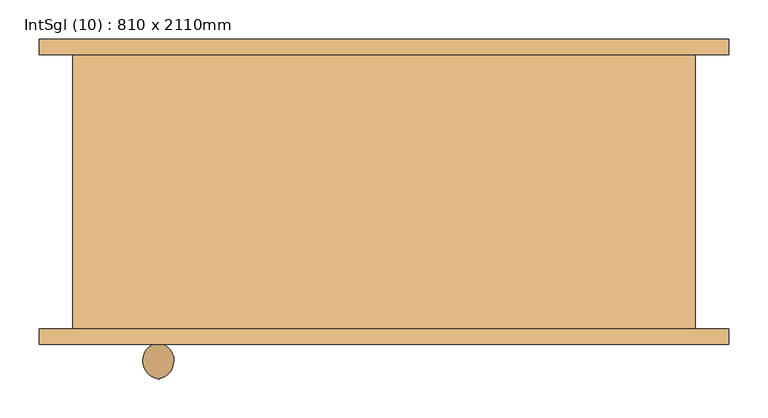
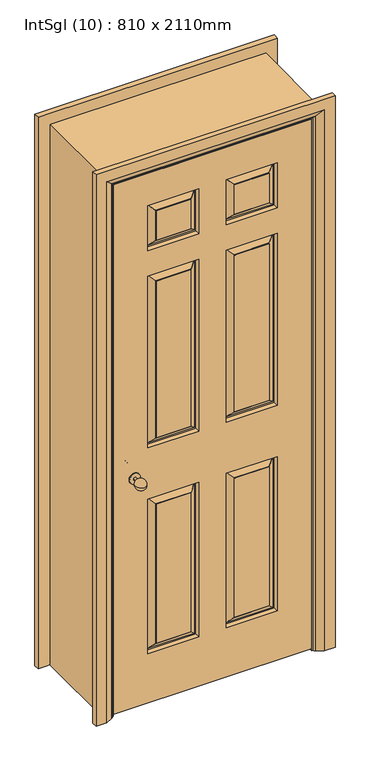
"""IFC4 building model written with IfcOpenShell, lengths in millimetres: door geometry, IntSgl (10) : 810 x 2110mm."""

from ifc_helpers import new_model, si_unit, point, frame, origin, place, context, project, spatial, polyline, circle_curve, ellipse_curve, trimmed, outline, extrude, faceted_brep, source, transform, mapped, element, save
from ifc_brep_helpers import plane_surface, cylinder_surface, revolved_surface, advanced_brep


def intsgl_10_810_x_2110mm_217d45f9(model_context):
    return source(origin(), model_context, "Body", "SolidModel", [
        advanced_brep(
        [(-283.0, -118.0, 900.0), (-293.0, -118.0, 900.0), (-288.0, -73.562589, 900.0), (-283.0, -133.0, 900.0), (-293.0, -133.0, 900.0), (-308.0, -137.0, 900.0), (-268.0, -137.0, 900.0), (-308.0, -133.0, 900.0), (-268.0, -133.0, 900.0)],
        [
            (0, 1, circle_curve(frame((-288.0, -118.0, 900.0), z_axis=(0.0, 1.0, 0.0), x_axis=(-1.0, 0.0, 0.0)), 5.0)),
            (1, 2, circle_curve(frame((-284.8115138, -96.4213505, 900.0), z_axis=(0.0, 0.0, -1.0), x_axis=(0.0, -1.0, 0.0)), 23.0800654)),
            (2, 0, circle_curve(frame((-291.1884862, -96.4213505, 900.0), z_axis=(0.0, 0.0, -1.0), x_axis=(0.0, -1.0, 0.0)), 23.0800654)),
            (1, 0, circle_curve(frame((-288.0, -118.0, 900.0), z_axis=(0.0, 1.0, 0.0), x_axis=(-1.0, 0.0, 0.0)), 5.0)),
            (0, 3),
            (3, 4, circle_curve(frame((-288.0, -133.0, 900.0), z_axis=(0.0, 1.0, 0.0), x_axis=(-1.0, 0.0, 0.0)), 5.0)),
            (4, 1),
            (4, 3, circle_curve(frame((-288.0, -133.0, 900.0), z_axis=(0.0, 1.0, 0.0), x_axis=(-1.0, 0.0, 0.0)), 5.0)),
            (5, 6, circle_curve(frame((-288.0, -137.0, 900.0), z_axis=(0.0, -1.0, 0.0), x_axis=(1.0, 0.0, 0.0)), 20.0)),
            (6, 5, circle_curve(frame((-288.0, -137.0, 900.0), z_axis=(0.0, -1.0, 0.0), x_axis=(1.0, 0.0, 0.0)), 20.0)),
            (7, 8, circle_curve(frame((-288.0, -133.0, 900.0), z_axis=(0.0, 1.0, 0.0), x_axis=(1.0, 0.0, 0.0)), 20.0)),
            (8, 7, circle_curve(frame((-288.0, -133.0, 900.0), z_axis=(0.0, 1.0, 0.0), x_axis=(1.0, 0.0, 0.0)), 20.0)),
            (5, 7),
            (8, 6),
        ],
        [
            revolved_surface(trimmed(ellipse_curve(frame((-284.8115138, -96.4213505, 900.0), z_axis=(0.0, 0.0, 1.0), x_axis=(0.0, -1.0, 0.0)), 23.0800654, 23.0800654), [point((-288.0, -73.562589, 900.0))], [point((-293.0, -118.0, 900.0))], True, "CARTESIAN"), (-288.0, -133.0, 900.0), (0.0, -1.0, 0.0)),
            cylinder_surface(frame((-288.0, -133.0, 900.0), z_axis=(0.0, -1.0, 0.0), x_axis=(-1.0, 0.0, 0.0)), 5.0),
            plane_surface(frame((-268.0, -137.0, 900.0), z_axis=(0.0, -1.0, 0.0), x_axis=(0.0, 0.0, 1.0))),
            plane_surface(frame((-268.0, -133.0, 900.0), z_axis=(0.0, 1.0, 0.0), x_axis=(0.0, 0.0, -1.0))),
            cylinder_surface(frame((-288.0, -133.0, 900.0), z_axis=(0.0, -1.0, 0.0), x_axis=(1.0, 0.0, 0.0)), 20.0),
        ],
        [
            (0, [[1, 2, 3]]),
            (0, [[-2, 4, -3]]),
            (1, [[-1, 5, 6, 7]]),
            (1, [[-4, -7, 8, -5]]),
            (2, [[9, 10]]),
            (3, [[11, 12], [-6, -8]]),
            (4, [[-9, 13, -12, 14]]),
            (4, [[-10, -14, -11, -13]]),
        ],
    ),
        advanced_brep(
        [(-283.0, -194.0, 900.0), (-288.0, -238.437411, 900.0), (-293.0, -194.0, 900.0), (-293.0, -179.0, 900.0), (-283.0, -179.0, 900.0), (-308.0, -175.0, 900.0), (-268.0, -175.0, 900.0), (-308.0, -179.0, 900.0), (-268.0, -179.0, 900.0)],
        [
            (0, 1, circle_curve(frame((-291.1884862, -215.5786495, 900.0), z_axis=(0.0, 0.0, -1.0), x_axis=(0.0, 1.0, 0.0)), 23.0800654)),
            (1, 2, circle_curve(frame((-284.8115138, -215.5786495, 900.0), z_axis=(0.0, 0.0, -1.0), x_axis=(0.0, 1.0, 0.0)), 23.0800654)),
            (2, 0, circle_curve(frame((-288.0, -194.0, 900.0), z_axis=(0.0, -1.0, 0.0), x_axis=(-1.0, 0.0, 0.0)), 5.0)),
            (0, 2, circle_curve(frame((-288.0, -194.0, 900.0), z_axis=(0.0, -1.0, 0.0), x_axis=(-1.0, 0.0, 0.0)), 5.0)),
            (2, 3),
            (3, 4, circle_curve(frame((-288.0, -179.0, 900.0), z_axis=(0.0, -1.0, 0.0), x_axis=(-1.0, 0.0, 0.0)), 5.0)),
            (4, 0),
            (4, 3, circle_curve(frame((-288.0, -179.0, 900.0), z_axis=(0.0, -1.0, 0.0), x_axis=(-1.0, 0.0, 0.0)), 5.0)),
            (5, 6, circle_curve(frame((-288.0, -175.0, 900.0), z_axis=(0.0, 1.0, 0.0), x_axis=(1.0, 0.0, 0.0)), 20.0)),
            (6, 5, circle_curve(frame((-288.0, -175.0, 900.0), z_axis=(0.0, 1.0, 0.0), x_axis=(1.0, 0.0, 0.0)), 20.0)),
            (7, 8, circle_curve(frame((-288.0, -179.0, 900.0), z_axis=(0.0, -1.0, 0.0), x_axis=(1.0, 0.0, 0.0)), 20.0)),
            (8, 7, circle_curve(frame((-288.0, -179.0, 900.0), z_axis=(0.0, -1.0, 0.0), x_axis=(1.0, 0.0, 0.0)), 20.0)),
            (6, 8),
            (7, 5),
        ],
        [
            revolved_surface(trimmed(ellipse_curve(frame((-284.8115138, -215.5786495, 900.0), z_axis=(0.0, 0.0, -1.0), x_axis=(0.0, 1.0, 0.0)), 23.0800654, 23.0800654), [point((-288.0, -238.437411, 900.0))], [point((-293.0, -194.0, 900.0))], True, "CARTESIAN"), (-288.0, -179.0, 900.0), (0.0, 1.0, 0.0)),
            cylinder_surface(frame((-288.0, -179.0, 900.0), z_axis=(0.0, 1.0, 0.0), x_axis=(-1.0, 0.0, 0.0)), 5.0),
            plane_surface(frame((-268.0, -175.0, 900.0), z_axis=(0.0, 1.0, 0.0), x_axis=(0.0, 0.0, 1.0))),
            plane_surface(frame((-268.0, -179.0, 900.0), z_axis=(0.0, -1.0, 0.0), x_axis=(0.0, 0.0, -1.0))),
            cylinder_surface(frame((-288.0, -179.0, 900.0), z_axis=(0.0, 1.0, 0.0), x_axis=(1.0, 0.0, 0.0)), 20.0),
        ],
        [
            (0, [[1, 2, 3]]),
            (0, [[-1, 4, -2]]),
            (1, [[5, 6, 7, -3]]),
            (1, [[-7, 8, -5, -4]]),
            (2, [[9, 10]]),
            (3, [[11, 12], [-8, -6]]),
            (4, [[13, -11, 14, -10]]),
            (4, [[-14, -12, -13, -9]]),
        ],
    ),
        faceted_brep([(-363.0, -137.0, 2068.0), (363.0, -137.0, 2068.0), (363.0, -137.0, 8.0), (-363.0, -137.0, 8.0), (-50.0, -137.0, 800.0), (-238.0, -137.0, 800.0), (-238.0, -137.0, 200.0), (-50.0, -137.0, 200.0), (238.0, -137.0, 800.0), (50.0, -137.0, 800.0), (50.0, -137.0, 200.0), (238.0, -137.0, 200.0), (-50.0, -137.0, 1668.0), (-238.0, -137.0, 1668.0), (-238.0, -137.0, 1000.0), (-50.0, -137.0, 1000.0), (238.0, -137.0, 1668.0), (50.0, -137.0, 1668.0), (50.0, -137.0, 1000.0), (238.0, -137.0, 1000.0), (-50.0, -137.0, 1943.0), (-238.0, -137.0, 1943.0), (-238.0, -137.0, 1768.0), (-50.0, -137.0, 1768.0), (238.0, -137.0, 1943.0), (50.0, -137.0, 1943.0), (50.0, -137.0, 1768.0), (238.0, -137.0, 1768.0), (-80.0, -137.0, 230.0), (-208.0, -137.0, 230.0), (-208.0, -137.0, 770.0), (-80.0, -137.0, 770.0), (208.0, -137.0, 230.0), (80.0, -137.0, 230.0), (80.0, -137.0, 770.0), (208.0, -137.0, 770.0), (-80.0, -137.0, 1030.0), (-208.0, -137.0, 1030.0), (-208.0, -137.0, 1638.0), (-80.0, -137.0, 1638.0), (208.0, -137.0, 1030.0), (80.0, -137.0, 1030.0), (80.0, -137.0, 1638.0), (208.0, -137.0, 1638.0), (-80.0, -137.0, 1798.0), (-208.0, -137.0, 1798.0), (-208.0, -137.0, 1913.0), (-80.0, -137.0, 1913.0), (208.0, -137.0, 1798.0), (80.0, -137.0, 1798.0), (80.0, -137.0, 1913.0), (208.0, -137.0, 1913.0), (-363.0, -175.0, 2068.0), (-363.0, -175.0, 8.0), (363.0, -175.0, 8.0), (363.0, -175.0, 2068.0), (50.0, -175.0, 800.0), (238.0, -175.0, 800.0), (238.0, -175.0, 200.0), (50.0, -175.0, 200.0), (-238.0, -175.0, 800.0), (-50.0, -175.0, 800.0), (-50.0, -175.0, 200.0), (-238.0, -175.0, 200.0), (50.0, -175.0, 1668.0), (238.0, -175.0, 1668.0), (238.0, -175.0, 1000.0), (50.0, -175.0, 1000.0), (-238.0, -175.0, 1668.0), (-50.0, -175.0, 1668.0), (-50.0, -175.0, 1000.0), (-238.0, -175.0, 1000.0), (50.0, -175.0, 1943.0), (238.0, -175.0, 1943.0), (238.0, -175.0, 1768.0), (50.0, -175.0, 1768.0), (-238.0, -175.0, 1943.0), (-50.0, -175.0, 1943.0), (-50.0, -175.0, 1768.0), (-238.0, -175.0, 1768.0), (80.0, -175.0, 230.0), (208.0, -175.0, 230.0), (208.0, -175.0, 770.0), (80.0, -175.0, 770.0), (-208.0, -175.0, 230.0), (-80.0, -175.0, 230.0), (-80.0, -175.0, 770.0), (-208.0, -175.0, 770.0), (80.0, -175.0, 1030.0), (208.0, -175.0, 1030.0), (208.0, -175.0, 1638.0), (80.0, -175.0, 1638.0), (-208.0, -175.0, 1030.0), (-80.0, -175.0, 1030.0), (-80.0, -175.0, 1638.0), (-208.0, -175.0, 1638.0), (80.0, -175.0, 1798.0), (208.0, -175.0, 1798.0), (208.0, -175.0, 1913.0), (80.0, -175.0, 1913.0), (-208.0, -175.0, 1798.0), (-80.0, -175.0, 1798.0), (-80.0, -175.0, 1913.0), (-208.0, -175.0, 1913.0), (80.0, -174.0, 230.0), (80.0, -174.0, 770.0), (58.0, -160.0, 208.0), (78.0, -174.0, 228.0), (78.0, -174.0, 772.0), (58.0, -160.0, 792.0), (53.0, -160.0, 203.0), (53.0, -160.0, 797.0), (208.0, -174.0, 770.0), (210.0, -174.0, 772.0), (230.0, -160.0, 792.0), (235.0, -160.0, 797.0), (208.0, -174.0, 230.0), (210.0, -174.0, 228.0), (230.0, -160.0, 208.0), (235.0, -160.0, 203.0), (-208.0, -174.0, 230.0), (-208.0, -174.0, 770.0), (-230.0, -160.0, 208.0), (-210.0, -174.0, 228.0), (-210.0, -174.0, 772.0), (-230.0, -160.0, 792.0), (-235.0, -160.0, 203.0), (-235.0, -160.0, 797.0), (-80.0, -174.0, 770.0), (-78.0, -174.0, 772.0), (-58.0, -160.0, 792.0), (-53.0, -160.0, 797.0), (-80.0, -174.0, 230.0), (-78.0, -174.0, 228.0), (-58.0, -160.0, 208.0), (-53.0, -160.0, 203.0), (80.0, -174.0, 1030.0), (80.0, -174.0, 1638.0), (58.0, -160.0, 1008.0), (78.0, -174.0, 1028.0), (78.0, -174.0, 1640.0), (58.0, -160.0, 1660.0), (53.0, -160.0, 1003.0), (53.0, -160.0, 1665.0), (208.0, -174.0, 1638.0), (210.0, -174.0, 1640.0), (230.0, -160.0, 1660.0), (235.0, -160.0, 1665.0), (208.0, -174.0, 1030.0), (210.0, -174.0, 1028.0), (230.0, -160.0, 1008.0), (235.0, -160.0, 1003.0), (-208.0, -174.0, 1030.0), (-208.0, -174.0, 1638.0), (-230.0, -160.0, 1008.0), (-210.0, -174.0, 1028.0), (-210.0, -174.0, 1640.0), (-230.0, -160.0, 1660.0), (-235.0, -160.0, 1003.0), (-235.0, -160.0, 1665.0), (-80.0, -174.0, 1638.0), (-78.0, -174.0, 1640.0), (-58.0, -160.0, 1660.0), (-53.0, -160.0, 1665.0), (-80.0, -174.0, 1030.0), (-78.0, -174.0, 1028.0), (-58.0, -160.0, 1008.0), (-53.0, -160.0, 1003.0), (80.0, -174.0, 1798.0), (80.0, -174.0, 1913.0), (58.0, -160.0, 1776.0), (78.0, -174.0, 1796.0), (78.0, -174.0, 1915.0), (58.0, -160.0, 1935.0), (53.0, -160.0, 1771.0), (53.0, -160.0, 1940.0), (208.0, -174.0, 1913.0), (210.0, -174.0, 1915.0), (230.0, -160.0, 1935.0), (235.0, -160.0, 1940.0), (208.0, -174.0, 1798.0), (210.0, -174.0, 1796.0), (230.0, -160.0, 1776.0), (235.0, -160.0, 1771.0), (-208.0, -174.0, 1798.0), (-208.0, -174.0, 1913.0), (-230.0, -160.0, 1776.0), (-210.0, -174.0, 1796.0), (-210.0, -174.0, 1915.0), (-230.0, -160.0, 1935.0), (-235.0, -160.0, 1771.0), (-235.0, -160.0, 1940.0), (-80.0, -174.0, 1913.0), (-78.0, -174.0, 1915.0), (-58.0, -160.0, 1935.0), (-53.0, -160.0, 1940.0), (-80.0, -174.0, 1798.0), (-78.0, -174.0, 1796.0), (-58.0, -160.0, 1776.0), (-53.0, -160.0, 1771.0), (-80.0, -138.0, 230.0), (-80.0, -138.0, 770.0), (-58.0, -152.0, 208.0), (-78.0, -138.0, 228.0), (-78.0, -138.0, 772.0), (-58.0, -152.0, 792.0), (-53.0, -152.0, 203.0), (-53.0, -152.0, 797.0), (-208.0, -138.0, 770.0), (-210.0, -138.0, 772.0), (-230.0, -152.0, 792.0), (-235.0, -152.0, 797.0), (-208.0, -138.0, 230.0), (-210.0, -138.0, 228.0), (-230.0, -152.0, 208.0), (-235.0, -152.0, 203.0), (208.0, -138.0, 230.0), (208.0, -138.0, 770.0), (230.0, -152.0, 208.0), (210.0, -138.0, 228.0), (210.0, -138.0, 772.0), (230.0, -152.0, 792.0), (235.0, -152.0, 203.0), (235.0, -152.0, 797.0), (80.0, -138.0, 770.0), (78.0, -138.0, 772.0), (58.0, -152.0, 792.0), (53.0, -152.0, 797.0), (80.0, -138.0, 230.0), (78.0, -138.0, 228.0), (58.0, -152.0, 208.0), (53.0, -152.0, 203.0), (-80.0, -138.0, 1030.0), (-80.0, -138.0, 1638.0), (-58.0, -152.0, 1008.0), (-78.0, -138.0, 1028.0), (-78.0, -138.0, 1640.0), (-58.0, -152.0, 1660.0), (-53.0, -152.0, 1003.0), (-53.0, -152.0, 1665.0), (-208.0, -138.0, 1638.0), (-210.0, -138.0, 1640.0), (-230.0, -152.0, 1660.0), (-235.0, -152.0, 1665.0), (-208.0, -138.0, 1030.0), (-210.0, -138.0, 1028.0), (-230.0, -152.0, 1008.0), (-235.0, -152.0, 1003.0), (208.0, -138.0, 1030.0), (208.0, -138.0, 1638.0), (230.0, -152.0, 1008.0), (210.0, -138.0, 1028.0), (210.0, -138.0, 1640.0), (230.0, -152.0, 1660.0), (235.0, -152.0, 1003.0), (235.0, -152.0, 1665.0), (80.0, -138.0, 1638.0), (78.0, -138.0, 1640.0), (58.0, -152.0, 1660.0), (53.0, -152.0, 1665.0), (80.0, -138.0, 1030.0), (78.0, -138.0, 1028.0), (58.0, -152.0, 1008.0), (53.0, -152.0, 1003.0), (-80.0, -138.0, 1798.0), (-80.0, -138.0, 1913.0), (-58.0, -152.0, 1776.0), (-78.0, -138.0, 1796.0), (-78.0, -138.0, 1915.0), (-58.0, -152.0, 1935.0), (-53.0, -152.0, 1771.0), (-53.0, -152.0, 1940.0), (-208.0, -138.0, 1913.0), (-210.0, -138.0, 1915.0), (-230.0, -152.0, 1935.0), (-235.0, -152.0, 1940.0), (-208.0, -138.0, 1798.0), (-210.0, -138.0, 1796.0), (-230.0, -152.0, 1776.0), (-235.0, -152.0, 1771.0), (208.0, -138.0, 1798.0), (208.0, -138.0, 1913.0), (230.0, -152.0, 1776.0), (210.0, -138.0, 1796.0), (210.0, -138.0, 1915.0), (230.0, -152.0, 1935.0), (235.0, -152.0, 1771.0), (235.0, -152.0, 1940.0), (80.0, -138.0, 1913.0), (78.0, -138.0, 1915.0), (58.0, -152.0, 1935.0), (53.0, -152.0, 1940.0), (80.0, -138.0, 1798.0), (78.0, -138.0, 1796.0), (58.0, -152.0, 1776.0), (53.0, -152.0, 1771.0)], [[[0, 1, 2, 3], [4, 5, 6, 7], [8, 9, 10, 11], [12, 13, 14, 15], [16, 17, 18, 19], [20, 21, 22, 23], [24, 25, 26, 27]], [[28, 29, 30, 31]], [[32, 33, 34, 35]], [[36, 37, 38, 39]], [[40, 41, 42, 43]], [[44, 45, 46, 47]], [[48, 49, 50, 51]], [[52, 53, 54, 55], [56, 57, 58, 59], [60, 61, 62, 63], [64, 65, 66, 67], [68, 69, 70, 71], [72, 73, 74, 75], [76, 77, 78, 79]], [[80, 81, 82, 83]], [[84, 85, 86, 87]], [[88, 89, 90, 91]], [[92, 93, 94, 95]], [[96, 97, 98, 99]], [[100, 101, 102, 103]], [[3, 53, 52, 0]], [[2, 54, 53, 3]], [[1, 55, 54, 2]], [[0, 52, 55, 1]], [[104, 80, 83, 105]], [[106, 107, 108, 109]], [[56, 59, 110, 111]], [[83, 82, 112, 105]], [[108, 113, 114, 109]], [[111, 115, 57, 56]], [[82, 81, 116, 112]], [[113, 117, 118, 114]], [[115, 119, 58, 57]], [[104, 116, 81, 80]], [[107, 117, 113, 108], [105, 112, 116, 104]], [[106, 118, 117, 107]], [[110, 119, 115, 111], [109, 114, 118, 106]], [[59, 58, 119, 110]], [[120, 84, 87, 121]], [[122, 123, 124, 125]], [[60, 63, 126, 127]], [[87, 86, 128, 121]], [[124, 129, 130, 125]], [[127, 131, 61, 60]], [[86, 85, 132, 128]], [[129, 133, 134, 130]], [[131, 135, 62, 61]], [[120, 132, 85, 84]], [[123, 133, 129, 124], [121, 128, 132, 120]], [[122, 134, 133, 123]], [[126, 135, 131, 127], [125, 130, 134, 122]], [[63, 62, 135, 126]], [[136, 88, 91, 137]], [[138, 139, 140, 141]], [[64, 67, 142, 143]], [[91, 90, 144, 137]], [[140, 145, 146, 141]], [[143, 147, 65, 64]], [[90, 89, 148, 144]], [[145, 149, 150, 146]], [[147, 151, 66, 65]], [[136, 148, 89, 88]], [[139, 149, 145, 140], [137, 144, 148, 136]], [[138, 150, 149, 139]], [[142, 151, 147, 143], [141, 146, 150, 138]], [[67, 66, 151, 142]], [[152, 92, 95, 153]], [[154, 155, 156, 157]], [[68, 71, 158, 159]], [[95, 94, 160, 153]], [[156, 161, 162, 157]], [[159, 163, 69, 68]], [[94, 93, 164, 160]], [[161, 165, 166, 162]], [[163, 167, 70, 69]], [[152, 164, 93, 92]], [[155, 165, 161, 156], [153, 160, 164, 152]], [[154, 166, 165, 155]], [[158, 167, 163, 159], [157, 162, 166, 154]], [[71, 70, 167, 158]], [[168, 96, 99, 169]], [[170, 171, 172, 173]], [[72, 75, 174, 175]], [[99, 98, 176, 169]], [[172, 177, 178, 173]], [[175, 179, 73, 72]], [[98, 97, 180, 176]], [[177, 181, 182, 178]], [[179, 183, 74, 73]], [[168, 180, 97, 96]], [[171, 181, 177, 172], [169, 176, 180, 168]], [[170, 182, 181, 171]], [[174, 183, 179, 175], [173, 178, 182, 170]], [[75, 74, 183, 174]], [[184, 100, 103, 185]], [[186, 187, 188, 189]], [[76, 79, 190, 191]], [[103, 102, 192, 185]], [[188, 193, 194, 189]], [[191, 195, 77, 76]], [[102, 101, 196, 192]], [[193, 197, 198, 194]], [[195, 199, 78, 77]], [[184, 196, 101, 100]], [[187, 197, 193, 188], [185, 192, 196, 184]], [[186, 198, 197, 187]], [[190, 199, 195, 191], [189, 194, 198, 186]], [[79, 78, 199, 190]], [[200, 28, 31, 201]], [[202, 203, 204, 205]], [[4, 7, 206, 207]], [[31, 30, 208, 201]], [[204, 209, 210, 205]], [[207, 211, 5, 4]], [[30, 29, 212, 208]], [[209, 213, 214, 210]], [[211, 215, 6, 5]], [[200, 212, 29, 28]], [[203, 213, 209, 204], [201, 208, 212, 200]], [[202, 214, 213, 203]], [[206, 215, 211, 207], [205, 210, 214, 202]], [[7, 6, 215, 206]], [[216, 32, 35, 217]], [[218, 219, 220, 221]], [[8, 11, 222, 223]], [[35, 34, 224, 217]], [[220, 225, 226, 221]], [[223, 227, 9, 8]], [[34, 33, 228, 224]], [[225, 229, 230, 226]], [[227, 231, 10, 9]], [[216, 228, 33, 32]], [[219, 229, 225, 220], [217, 224, 228, 216]], [[218, 230, 229, 219]], [[222, 231, 227, 223], [221, 226, 230, 218]], [[11, 10, 231, 222]], [[232, 36, 39, 233]], [[234, 235, 236, 237]], [[12, 15, 238, 239]], [[39, 38, 240, 233]], [[236, 241, 242, 237]], [[239, 243, 13, 12]], [[38, 37, 244, 240]], [[241, 245, 246, 242]], [[243, 247, 14, 13]], [[232, 244, 37, 36]], [[235, 245, 241, 236], [233, 240, 244, 232]], [[234, 246, 245, 235]], [[238, 247, 243, 239], [237, 242, 246, 234]], [[15, 14, 247, 238]], [[248, 40, 43, 249]], [[250, 251, 252, 253]], [[16, 19, 254, 255]], [[43, 42, 256, 249]], [[252, 257, 258, 253]], [[255, 259, 17, 16]], [[42, 41, 260, 256]], [[257, 261, 262, 258]], [[259, 263, 18, 17]], [[248, 260, 41, 40]], [[251, 261, 257, 252], [249, 256, 260, 248]], [[250, 262, 261, 251]], [[254, 263, 259, 255], [253, 258, 262, 250]], [[19, 18, 263, 254]], [[264, 44, 47, 265]], [[266, 267, 268, 269]], [[20, 23, 270, 271]], [[47, 46, 272, 265]], [[268, 273, 274, 269]], [[271, 275, 21, 20]], [[46, 45, 276, 272]], [[273, 277, 278, 274]], [[275, 279, 22, 21]], [[264, 276, 45, 44]], [[267, 277, 273, 268], [265, 272, 276, 264]], [[266, 278, 277, 267]], [[270, 279, 275, 271], [269, 274, 278, 266]], [[23, 22, 279, 270]], [[280, 48, 51, 281]], [[282, 283, 284, 285]], [[24, 27, 286, 287]], [[51, 50, 288, 281]], [[284, 289, 290, 285]], [[287, 291, 25, 24]], [[50, 49, 292, 288]], [[289, 293, 294, 290]], [[291, 295, 26, 25]], [[280, 292, 49, 48]], [[283, 293, 289, 284], [281, 288, 292, 280]], [[282, 294, 293, 283]], [[286, 295, 291, 287], [285, 290, 294, 282]], [[27, 26, 295, 286]]]),
        advanced_brep(
        [(440.0, -195.0, 0.0), (400.0, -195.0, 0.0), (374.0, -181.0, 0.0), (370.0, -175.0, 0.0), (440.0, -175.0, 0.0), (440.0, -175.0, 2145.0), (440.0, -195.0, 2145.0), (370.0, -175.0, 2075.0), (-370.0, -175.0, 2075.0), (-370.0, -175.0, 0.0), (-440.0, -175.0, 0.0), (-440.0, -175.0, 2145.0), (374.0, -181.0, 2079.0), (400.0, -195.0, 2105.0), (-440.0, -195.0, 2145.0), (-440.0, -195.0, 0.0), (-400.0, -195.0, 0.0), (-400.0, -195.0, 2105.0), (-374.0, -181.0, 0.0), (-374.0, -181.0, 2079.0)],
        [
            (0, 1),
            (1, 2),
            (2, 3, circle_curve(frame((378.0, -174.0, 0.0), z_axis=(0.0, 0.0, -1.0), x_axis=(1.0, 0.0, 0.0)), 8.0622577)),
            (3, 4),
            (4, 0),
            (4, 5),
            (5, 6),
            (6, 0),
            (3, 7),
            (7, 8),
            (8, 9),
            (9, 10),
            (10, 11),
            (11, 5),
            (2, 12),
            (12, 7, ellipse_curve(frame((378.0, -174.0, 2083.0), z_axis=(0.7071067811865475, 0.0, -0.7071067811865475), x_axis=(-0.7071067811865474, 0.0, -0.7071067811865476)), 11.4017543, 8.0622577)),
            (1, 13),
            (13, 12),
            (6, 14),
            (14, 15),
            (15, 16),
            (16, 17),
            (17, 13),
            (10, 15),
            (14, 11),
            (9, 18, circle_curve(frame((-378.0, -174.0, 0.0), z_axis=(0.0, 0.0, -1.0), x_axis=(-1.0, 0.0, 0.0)), 8.0622577)),
            (18, 16),
            (19, 18),
            (8, 19, ellipse_curve(frame((-378.0, -174.0, 2083.0), z_axis=(-0.7071067811865475, 0.0, -0.7071067811865475), x_axis=(-0.7071067811865474, 0.0, 0.7071067811865476)), 11.4017543, 8.0622577)),
            (19, 17),
            (12, 19),
        ],
        [
            plane_surface(frame((370.0, -175.0, 0.0), z_axis=(0.0, 0.0, -1.0), x_axis=(0.0, -1.0, 0.0))),
            plane_surface(frame((440.0, -195.0, 0.0), z_axis=(1.0, 0.0, 0.0), x_axis=(0.0, 0.0, 1.0))),
            plane_surface(frame((440.0, -175.0, 0.0), z_axis=(0.0, 1.0, 0.0), x_axis=(0.0, 0.0, 1.0))),
            cylinder_surface(frame((378.0, -174.0, 0.0), z_axis=(0.0, 0.0, -1.0), x_axis=(1.0, 0.0, 0.0)), 8.0622577),
            plane_surface(frame((374.0, -181.0, 0.0), z_axis=(-0.4740998230350183, -0.8804710999221749, 0.0), x_axis=(0.0, 0.0, 1.0))),
            plane_surface(frame((400.0, -195.0, 0.0), z_axis=(0.0, -1.0, 0.0), x_axis=(0.0, 0.0, 1.0))),
            plane_surface(frame((-440.0, -195.0, 2145.0), z_axis=(-1.0, 0.0, 0.0), x_axis=(0.0, 0.0, -1.0))),
            plane_surface(frame((-370.0, -175.0, 0.0), z_axis=(0.0, 0.0, -1.0), x_axis=(0.0, -1.0, 0.0))),
            cylinder_surface(frame((-378.0, -174.0, 2075.0), z_axis=(0.0, 0.0, 1.0), x_axis=(-1.0, 0.0, 0.0)), 8.0622577),
            plane_surface(frame((-374.0, -181.0, 2079.0), z_axis=(0.4740998230350183, -0.8804710999221749, 0.0), x_axis=(0.0, 0.0, -1.0))),
            plane_surface(frame((440.0, -195.0, 2145.0), z_axis=(0.0, 0.0, 1.0), x_axis=(-1.0, 0.0, 0.0))),
            cylinder_surface(frame((370.0, -174.0, 2083.0), z_axis=(1.0, 0.0, 0.0), x_axis=(0.0, 0.0, 1.0)), 8.0622577),
            plane_surface(frame((374.0, -181.0, 2079.0), z_axis=(0.0, -0.8804710999221749, -0.4740998230350183), x_axis=(-1.0, 0.0, 0.0))),
        ],
        [
            (0, [[1, 2, 3, 4, 5]]),
            (1, [[6, 7, 8, -5]]),
            (2, [[9, 10, 11, 12, 13, 14, -6, -4]]),
            (3, [[15, 16, -9, -3]]),
            (4, [[17, 18, -15, -2]]),
            (5, [[-8, 19, 20, 21, 22, 23, -17, -1]]),
            (6, [[-13, 24, -20, 25]]),
            (7, [[-24, -12, 26, 27, -21]]),
            (8, [[28, -26, -11, 29]]),
            (9, [[-22, -27, -28, 30]]),
            (10, [[-14, -25, -19, -7]]),
            (11, [[31, -29, -10, -16]]),
            (12, [[-23, -30, -31, -18]]),
        ],
    ),
        advanced_brep(
        [(-440.0, 195.0, 0.0), (-400.0, 195.0, 0.0), (-374.0, 181.0, 0.0), (-370.0, 175.0, 0.0), (-440.0, 175.0, 0.0), (-440.0, 175.0, 2145.0), (-440.0, 195.0, 2145.0), (-370.0, 175.0, 2075.0), (370.0, 175.0, 2075.0), (370.0, 175.0, 0.0), (440.0, 175.0, 0.0), (440.0, 175.0, 2145.0), (-374.0, 181.0, 2079.0), (-400.0, 195.0, 2105.0), (440.0, 195.0, 2145.0), (440.0, 195.0, 0.0), (400.0, 195.0, 0.0), (400.0, 195.0, 2105.0), (374.0, 181.0, 0.0), (374.0, 181.0, 2079.0)],
        [
            (0, 1),
            (1, 2),
            (2, 3, circle_curve(frame((-378.0, 174.0, 0.0), z_axis=(0.0, 0.0, -1.0), x_axis=(-1.0, 0.0, 0.0)), 8.0622577)),
            (3, 4),
            (4, 0),
            (4, 5),
            (5, 6),
            (6, 0),
            (3, 7),
            (7, 8),
            (8, 9),
            (9, 10),
            (10, 11),
            (11, 5),
            (2, 12),
            (12, 7, ellipse_curve(frame((-378.0, 174.0, 2083.0), z_axis=(-0.7071067811865475, 0.0, -0.7071067811865475), x_axis=(0.7071067811865474, 0.0, -0.7071067811865476)), 11.4017543, 8.0622577)),
            (1, 13),
            (13, 12),
            (6, 14),
            (14, 15),
            (15, 16),
            (16, 17),
            (17, 13),
            (10, 15),
            (14, 11),
            (9, 18, circle_curve(frame((378.0, 174.0, 0.0), z_axis=(0.0, 0.0, -1.0), x_axis=(1.0, 0.0, 0.0)), 8.0622577)),
            (18, 16),
            (19, 18),
            (8, 19, ellipse_curve(frame((378.0, 174.0, 2083.0), z_axis=(0.7071067811865475, 0.0, -0.7071067811865475), x_axis=(0.7071067811865474, 0.0, 0.7071067811865476)), 11.4017543, 8.0622577)),
            (19, 17),
            (12, 19),
        ],
        [
            plane_surface(frame((-370.0, 175.0, 0.0), z_axis=(0.0, 0.0, -1.0), x_axis=(0.0, 1.0, 0.0))),
            plane_surface(frame((-440.0, 195.0, 0.0), z_axis=(-1.0, 0.0, 0.0), x_axis=(0.0, 0.0, 1.0))),
            plane_surface(frame((-440.0, 175.0, 0.0), z_axis=(0.0, -1.0, 0.0), x_axis=(0.0, 0.0, 1.0))),
            cylinder_surface(frame((-378.0, 174.0, 0.0), z_axis=(0.0, 0.0, -1.0), x_axis=(-1.0, 0.0, 0.0)), 8.0622577),
            plane_surface(frame((-374.0, 181.0, 0.0), z_axis=(0.4740998230350183, 0.8804710999221749, 0.0), x_axis=(0.0, 0.0, 1.0))),
            plane_surface(frame((-400.0, 195.0, 0.0), z_axis=(0.0, 1.0, 0.0), x_axis=(0.0, 0.0, 1.0))),
            plane_surface(frame((440.0, 195.0, 2145.0), z_axis=(1.0, 0.0, 0.0), x_axis=(0.0, 0.0, -1.0))),
            plane_surface(frame((370.0, 175.0, 0.0), z_axis=(0.0, 0.0, -1.0), x_axis=(0.0, 1.0, 0.0))),
            cylinder_surface(frame((378.0, 174.0, 2075.0), z_axis=(0.0, 0.0, 1.0), x_axis=(1.0, 0.0, 0.0)), 8.0622577),
            plane_surface(frame((374.0, 181.0, 2079.0), z_axis=(-0.4740998230350183, 0.8804710999221749, 0.0), x_axis=(0.0, 0.0, -1.0))),
            plane_surface(frame((-440.0, 195.0, 2145.0), z_axis=(0.0, 0.0, 1.0), x_axis=(1.0, 0.0, 0.0))),
            cylinder_surface(frame((-370.0, 174.0, 2083.0), z_axis=(-1.0, 0.0, 0.0), x_axis=(0.0, 0.0, 1.0)), 8.0622577),
            plane_surface(frame((-374.0, 181.0, 2079.0), z_axis=(0.0, 0.8804710999221749, -0.4740998230350183), x_axis=(1.0, 0.0, 0.0))),
        ],
        [
            (0, [[1, 2, 3, 4, 5]]),
            (1, [[6, 7, 8, -5]]),
            (2, [[9, 10, 11, 12, 13, 14, -6, -4]]),
            (3, [[15, 16, -9, -3]]),
            (4, [[17, 18, -15, -2]]),
            (5, [[-8, 19, 20, 21, 22, 23, -17, -1]]),
            (6, [[-13, 24, -20, 25]]),
            (7, [[-24, -12, 26, 27, -21]]),
            (8, [[28, -26, -11, 29]]),
            (9, [[-22, -27, -28, 30]]),
            (10, [[-14, -25, -19, -7]]),
            (11, [[31, -29, -10, -16]]),
            (12, [[-23, -30, -31, -18]]),
        ],
    ),
        extrude(outline(polyline([(0.0, -346.0), (2051.0, -346.0), (2051.0, 346.0), (0.0, 346.0), (0.0, 365.0), (2070.0, 365.0), (2070.0, -365.0), (0.0, -365.0), (0.0, -346.0)])), frame((0.0, -135.0, 0.0), z_axis=(0.0, 1.0, 0.0), x_axis=(0.0, 0.0, 1.0)), (0.0, 0.0, 1.0), 32.0),
        faceted_brep([(-365.0, -175.0, 0.0), (-397.0, -175.0, 0.0), (-397.0, 175.0, 0.0), (-365.0, 175.0, 0.0), (-365.0, 175.0, 2070.0), (-365.0, -175.0, 2070.0), (-397.0, 175.0, 2102.0), (-397.0, -175.0, 2102.0), (365.0, -175.0, 0.0), (365.0, 175.0, 0.0), (397.0, 175.0, 0.0), (397.0, -175.0, 0.0), (365.0, -175.0, 2070.0), (397.0, -175.0, 2102.0), (397.0, 175.0, 2102.0), (365.0, 175.0, 2070.0)], [[[0, 1, 2, 3]], [[3, 4, 5, 0]], [[2, 6, 4, 3]], [[1, 7, 6, 2]], [[0, 5, 7, 1]], [[8, 9, 10, 11]], [[12, 8, 11, 13]], [[13, 11, 10, 14]], [[14, 10, 9, 15]], [[15, 9, 8, 12]], [[4, 15, 12, 5]], [[6, 14, 15, 4]], [[7, 13, 14, 6]], [[5, 12, 13, 7]]]),
    ])


if __name__ == "__main__":
    model = new_model("IFC4")
    model_context = context("Model", 3, world=origin())
    ifc_project = project(units=[si_unit("LENGTHUNIT", "METRE", prefix="MILLI")], contexts=[model_context])
    site = spatial("IfcSite", under=ifc_project)
    building = spatial("IfcBuilding", under=site)
    placement = place(None, origin())
    intsgl_10_810_x_2110mm_shape = intsgl_10_810_x_2110mm_217d45f9(model_context)
    element("IfcDoor", 1, ObjectType="IntSgl (10) : 810 x 2110mm", at=placement, inside=building, context=model_context, shape_type="MappedRepresentation", body=[
        mapped(intsgl_10_810_x_2110mm_shape, transform((0.0, 0.0, 0.0), x_axis=(1.0, 0.0, 0.0), y_axis=(0.0, 1.0, 0.0), z_axis=(0.0, 0.0, 1.0))),
    ])
    save(model, "model.ifc")

# Revit data of these elements
# Type "IntSgl (10) : 810 x 2110mm"
#   Type Mark = "9"
#   Type Comments = "Internal Single"
#   Operation = "SingleSwingRight"
#   Manufacturer = "Revit"
#   Keynote = "L20"
#   Description = "Internal Single Door"
#   UnderCut = 8 mm
#   Tolerance = 2 mm
#   Thickness = 38 mm
#   Structural Tolerance = 8 mm
#   StopDepth = 32 mm
#   Stop Thickness = 19 mm
#   Stile Top Rail = 125 mm
#   Stile Shutting = 125 mm
#   Stile Muntin Rail = 100 mm
#   Stile Lock Rail = 200 mm
#   Stile Intermediate/Frieze = 100 mm
#   Stile Hanging = 125 mm
#   Stile Bottom Rail = 200 mm
#   Rough Width = 810 mm
#   Rough Height = 2110 mm
#   Height to Top Lock Rail = 1000 mm
#   Handle Z Distance = 900 mm
#   Handle X Distance = 75 mm
#   Frame Thickness = 32 mm
#   Door Panel Width = 726 mm
#   Height = 2110 mm
#   Width = 810 mm
#   Door Panel Thickness = 38 mm
#   Door Panel Offset = 0 mm
#   Door Panel Height = 2060 mm
#   Architrave Setback = 5 mm
#   Vis - Ironmongery = yes
#   Material Ironmongery = Door - Panel
#   Material Frame = Door - Frame/Mullion
#   Material Door = Door - Panel
#   Material Architrave = Door - Architrave
#   Function = (empty or 0)
#   Wall Closure = (empty or 0)
# Element 1 (IfcDoor, "IntSgl (10) : 810 x 2110mm")
#   Materials on its faces: "Door - Panel", "Door - Architrave", "Door - Frame/Mullion"
# Materials
#   "Door - Panel": class "Wood", colour RGB 210 159 95, transparency 0
#   "Door - Frame/Mullion": class "Wood", colour RGB 212 179 113, transparency 0
#   "Door - Architrave": class "Wood", colour RGB 154 90 5, transparency 0
